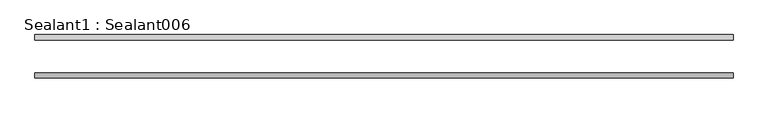
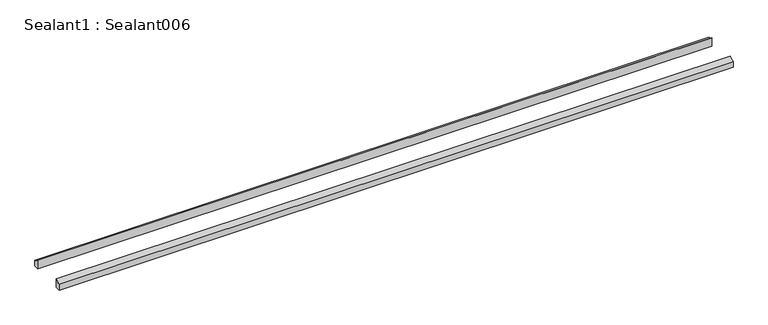
"""IFC4 building model written with IfcOpenShell, lengths in millimetres: proxy geometry, Sealant1 : Sealant006."""

import ifcopenshell
import ifcopenshell.guid

model = None  # the IFC model being written
_history = None  # IfcOwnerHistory: only IFC2X3 demands one
_inside = {}  # id of a spatial element -> (the spatial element, [elements in it])
_under = {}  # id of a project, library or spatial element -> (it, [spatial elements below it])
_declared = {}  # id of a project -> (the project, [libraries it declares])
_typed = {}  # id of a type object -> (the type object, [elements of that type])
_made_of = {}  # id of a material, layer set ... -> (it, [elements and type objects made of it])


def new_model(schema):
    """Start an empty IFC model of exactly this schema.

    Asked for "IFC4X3", IfcOpenShell would pick the latest addendum, in which some entities
    have other attributes; the version numbers below select the first issue.
    IFC2X3 requires an IfcOwnerHistory on every rooted entity: one is made here for all.
    """
    global model, _history
    if schema == "IFC4X3":
        model = ifcopenshell.file(schema_version=(4, 3, 0, 0))
    else:
        model = ifcopenshell.file(schema=schema)
    _inside.clear()
    _under.clear()
    _declared.clear()
    _typed.clear()
    _made_of.clear()
    _history = None
    if model.schema == "IFC2X3":
        org = make("IfcOrganization", Name="unknown")
        user = make(
            "IfcPersonAndOrganization",
            ThePerson=make("IfcPerson", FamilyName="unknown"),
            TheOrganization=org,
        )
        app = make(
            "IfcApplication",
            ApplicationDeveloper=org,
            Version="unknown",
            ApplicationFullName="unknown",
            ApplicationIdentifier="unknown",
        )
        _history = make(
            "IfcOwnerHistory",
            OwningUser=user,
            OwningApplication=app,
            ChangeAction="ADDED",
            CreationDate=0,
        )
    return model


def make(cls, **values):
    """One entity of the class cls with the attributes given. An attribute that is None is left unset."""
    return model.create_entity(
        cls, **{name: value for name, value in values.items() if value is not None}
    )


def rooted(cls, **values):
    """An entity with a GlobalId (a new one), such as an element, a storey or a relation."""
    return make(cls, GlobalId=ifcopenshell.guid.new(), OwnerHistory=_history, **values)


def si_unit(unit_type, name, prefix=None):
    """IfcSIUnit, for example si_unit("LENGTHUNIT", "METRE", prefix="MILLI")."""
    return make("IfcSIUnit", UnitType=unit_type, Prefix=prefix, Name=name)


def assignment(units):
    """IfcUnitAssignment: the units of a project."""
    return None if units is None else make("IfcUnitAssignment", Units=units)


def point(xyz):
    """IfcCartesianPoint."""
    return None if xyz is None else make("IfcCartesianPoint", Coordinates=xyz)


def direction(xyz):
    """IfcDirection."""
    return None if xyz is None else make("IfcDirection", DirectionRatios=xyz)


def frame(location, z_axis=None, x_axis=None):
    """IfcAxis2Placement3D, a coordinate frame: its origin and axes. An axis left out is left unset."""
    return make(
        "IfcAxis2Placement3D",
        Location=point(location),
        Axis=direction(z_axis),
        RefDirection=direction(x_axis),
    )


def frame_2d(location, x_axis=None):
    """IfcAxis2Placement2D, a coordinate frame in the plane: its origin and x axis."""
    return make(
        "IfcAxis2Placement2D", Location=point(location), RefDirection=direction(x_axis)
    )


def origin():
    """The frame at (0, 0, 0) with its axes left unset."""
    return frame((0.0, 0.0, 0.0))


def place(relative_to, where):
    """IfcLocalPlacement: puts the frame where relative to a parent placement (None: the world)."""
    return make(
        "IfcLocalPlacement", PlacementRelTo=relative_to, RelativePlacement=where
    )


def context(
    kind, dimensions, precision=None, world=None, true_north=None, identifier=None
):
    """IfcGeometricRepresentationContext, for example the 3D "Model" context."""
    return make(
        "IfcGeometricRepresentationContext",
        ContextIdentifier=identifier,
        ContextType=kind,
        CoordinateSpaceDimension=dimensions,
        Precision=precision,
        WorldCoordinateSystem=world,
        TrueNorth=true_north,
    )


def project(units=None, contexts=None):
    """IfcProject with its units and contexts."""
    return rooted(
        "IfcProject",
        Name="project",
        RepresentationContexts=contexts,
        UnitsInContext=assignment(units),
    )


def spatial(cls, under=None, at=None, **own):
    """A site, building, storey or space (cls), placed at a placement, below another one or the project."""
    s = rooted(cls, ObjectPlacement=at, **own)
    if under is not None:
        _under.setdefault(under.id(), (under, []))[1].append(s)
    return s


def polyline(points):
    """IfcPolyline through the points."""
    return make("IfcPolyline", Points=[point(p) for p in points])


def circle_curve(where, radius):
    """IfcCircle in the frame where."""
    return make("IfcCircle", Position=where, Radius=radius)


def trimmed(basis, trim1, trim2, sense, master):
    """IfcTrimmedCurve: the piece of a basis curve between two trims."""
    return make(
        "IfcTrimmedCurve",
        BasisCurve=basis,
        Trim1=trim1,
        Trim2=trim2,
        SenseAgreement=sense,
        MasterRepresentation=master,
    )


def segment(curve, same_sense, transition):
    """IfcCompositeCurveSegment."""
    return make(
        "IfcCompositeCurveSegment",
        Transition=transition,
        SameSense=same_sense,
        ParentCurve=curve,
    )


def composite_curve(segments, self_intersect=None):
    """IfcCompositeCurve: segments joined end to end."""
    return make("IfcCompositeCurve", Segments=segments, SelfIntersect=self_intersect)


def outline(outer, holes=None, kind="AREA"):
    """IfcArbitraryClosedProfileDef: a profile drawn as a closed curve; with holes, ...WithVoids."""
    if holes is None:
        return make("IfcArbitraryClosedProfileDef", ProfileType=kind, OuterCurve=outer)
    return make(
        "IfcArbitraryProfileDefWithVoids",
        ProfileType=kind,
        OuterCurve=outer,
        InnerCurves=holes,
    )


def extrude(swept, where, along, depth):
    """IfcExtrudedAreaSolid: the profile swept, set in the frame where, extruded along a direction by depth."""
    return make(
        "IfcExtrudedAreaSolid",
        SweptArea=swept,
        Position=where,
        ExtrudedDirection=direction(along),
        Depth=depth,
    )


def shape(context_of_items, identifier, shape_type, items):
    """IfcShapeRepresentation: the items that make up one representation, for example the "Body"."""
    return make(
        "IfcShapeRepresentation",
        ContextOfItems=context_of_items,
        RepresentationIdentifier=identifier,
        RepresentationType=shape_type,
        Items=items,
    )


def source(mapping_origin, context_of_items, identifier, shape_type, items):
    """IfcRepresentationMap: a shape defined once, which mapped items show again and again."""
    return make(
        "IfcRepresentationMap",
        MappingOrigin=mapping_origin,
        MappedRepresentation=shape(context_of_items, identifier, shape_type, items),
    )


def transform(
    local_origin,
    x_axis=None,
    y_axis=None,
    z_axis=None,
    scale=None,
    scale2=None,
    scale3=None,
    uniform=True,
):
    """IfcCartesianTransformationOperator3D, or its non-uniform kind. x_axis, y_axis, z_axis: its Axis1, 2, 3."""
    if uniform:
        return make(
            "IfcCartesianTransformationOperator3D",
            Axis1=direction(x_axis),
            Axis2=direction(y_axis),
            LocalOrigin=point(local_origin),
            Scale=scale,
            Axis3=direction(z_axis),
        )
    return make(
        "IfcCartesianTransformationOperator3DnonUniform",
        Axis1=direction(x_axis),
        Axis2=direction(y_axis),
        LocalOrigin=point(local_origin),
        Scale=scale,
        Axis3=direction(z_axis),
        Scale2=scale2,
        Scale3=scale3,
    )


def mapped(mapping_source, mapping_target):
    """IfcMappedItem: shows the shape of a source again, moved by a transform."""
    return make(
        "IfcMappedItem", MappingSource=mapping_source, MappingTarget=mapping_target
    )


def made_of(thing, what):
    """Note that an element or type object is made of a material, layer set ...; save() writes the relation."""
    if what is not None:
        _made_of.setdefault(what.id(), (what, []))[1].append(thing)
    return thing


def element(
    cls,
    number,
    at=None,
    inside=None,
    cuts=None,
    type_object=None,
    material=None,
    context=None,
    identifier="Body",
    shape_type=None,
    held_by="IfcProductDefinitionShape",
    body=None,
    shapes=None,
    **own,
):
    """One element of the class cls, such as IfcWall. Its Tag is "e" and its number.

    at: its placement. inside: the storey or other place that contains it. cuts: it is an
    opening in that element (IfcRelVoidsElement). A single representation is given by context,
    identifier, shape_type and body (its items); several are given by shapes. held_by: the class
    of the entity that holds the representations. save() writes the other relations.
    """
    e = rooted(cls, Tag="e%d" % number, ObjectPlacement=at, **own)
    if body is not None:
        shapes = [shape(context, identifier, shape_type, body)]
    if shapes is not None:
        e.Representation = make(held_by, Representations=shapes)
    if inside is not None:
        _inside.setdefault(inside.id(), (inside, []))[1].append(e)
    if cuts is not None:
        rooted(
            "IfcRelVoidsElement", RelatingBuildingElement=cuts, RelatedOpeningElement=e
        )
    if type_object is not None:
        _typed.setdefault(type_object.id(), (type_object, []))[1].append(e)
    return made_of(e, material)


def aggregate(whole, parts):
    """IfcRelAggregates: a whole, such as a stair, and the parts it consists of."""
    return rooted("IfcRelAggregates", RelatingObject=whole, RelatedObjects=parts)


def save(model, path):
    """Write the relations noted so far, then the file.

    IfcRelAggregates (storeys below a building ...), IfcRelContainedInSpatialStructure (elements
    in a storey), IfcRelDefinesByType, IfcRelAssociatesMaterial and IfcRelDeclares: one each for
    every whole, place, type object, material and project.
    """
    for whole, parts in _under.values():
        aggregate(whole, parts)
    for where, things in _inside.values():
        rooted(
            "IfcRelContainedInSpatialStructure",
            RelatedElements=things,
            RelatingStructure=where,
        )
    for kind, things in _typed.values():
        rooted("IfcRelDefinesByType", RelatedObjects=things, RelatingType=kind)
    for what, things in _made_of.values():
        rooted("IfcRelAssociatesMaterial", RelatedObjects=things, RelatingMaterial=what)
    for by, libraries in _declared.values():
        rooted("IfcRelDeclares", RelatingContext=by, RelatedDefinitions=libraries)
    model.write(path)


def sealant1_sealant006_b5695fb9(model_context):
    return source(origin(), model_context, "Body", "SweptSolid", [
        extrude(outline(composite_curve([segment(trimmed(circle_curve(frame_2d((9644.4481724, 39482.1594181)), 26.2617043), [point((9625.2926199, 39464.1943986))], [point((9640.2075717, 39456.2423499))], True, "CARTESIAN"), True, "CONTINUOUS"), segment(polyline([(9640.2075717, 39456.2423499), (9640.2075717, 39438.0491075), (9625.2926199, 39438.0491075), (9625.2926199, 39464.1943986)]), True, "CONTINUOUS")], self_intersect=False)), frame((-9232.0719278, 0.0, 0.0), z_axis=(1.0, 0.0, 0.0), x_axis=(0.0, 1.0, 0.0)), (0.0, 0.0, 1.0), 1999.85),
        extrude(outline(composite_curve([segment(polyline([(9530.5322891, 39464.1943986), (9530.5322891, 39438.0491075), (9515.6173373, 39438.0491075), (9515.6173373, 39456.2423499)]), True, "CONTINUOUS"), segment(trimmed(circle_curve(frame_2d((9511.3767366, 39482.1594181)), 26.2617043), [point((9515.6173373, 39456.2423499))], [point((9530.5322891, 39464.1943986))], True, "CARTESIAN"), True, "CONTINUOUS")], self_intersect=False)), frame((-9232.0719278, 0.0, 0.0), z_axis=(1.0, 0.0, 0.0), x_axis=(0.0, 1.0, 0.0)), (0.0, 0.0, 1.0), 1999.85),
    ])


if __name__ == "__main__":
    model = new_model("IFC4")
    model_context = context("Model", 3, world=origin())
    ifc_project = project(units=[si_unit("LENGTHUNIT", "METRE", prefix="MILLI")], contexts=[model_context])
    site = spatial("IfcSite", under=ifc_project)
    building = spatial("IfcBuilding", under=site)
    placement = place(None, origin())
    sealant1_sealant006_shape = sealant1_sealant006_b5695fb9(model_context)
    element("IfcBuildingElementProxy", 1, Name="Sealant1 : Sealant006", ObjectType="Sealant1 : Sealant006", at=placement, inside=building, context=model_context, shape_type="MappedRepresentation", body=[
        mapped(sealant1_sealant006_shape, transform((0.0, 0.0, 0.0), x_axis=(1.0, 0.0, 0.0), y_axis=(0.0, 1.0, 0.0), z_axis=(0.0, 0.0, 1.0))),
    ])
    save(model, "model.ifc")

# Revit data of these elements
# Type "Sealant1 : Sealant006"
#   NameOverride = "Sealant006"
# Element 1 (IfcBuildingElementProxy, "Sealant1 : Sealant006")
#   Materials on its faces: "SEALANT AND BACKER ROD WHERE NECESSARY"
# Materials
#   "SEALANT AND BACKER ROD WHERE NECESSARY": class "Unassigned", colour RGB 225 240 198, transparency 0, Cost = 0
